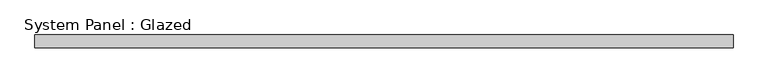
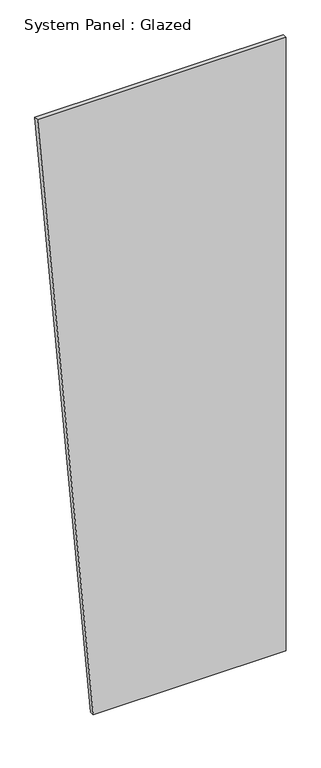
"""IFC4 building model written with IfcOpenShell, lengths in millimetres: plate geometry, System Panel : Glazed."""

import ifcopenshell
import ifcopenshell.guid

model = None  # the IFC model being written
_history = None  # IfcOwnerHistory: only IFC2X3 demands one
_inside = {}  # id of a spatial element -> (the spatial element, [elements in it])
_under = {}  # id of a project, library or spatial element -> (it, [spatial elements below it])
_declared = {}  # id of a project -> (the project, [libraries it declares])
_typed = {}  # id of a type object -> (the type object, [elements of that type])
_made_of = {}  # id of a material, layer set ... -> (it, [elements and type objects made of it])


def new_model(schema):
    """Start an empty IFC model of exactly this schema.

    Asked for "IFC4X3", IfcOpenShell would pick the latest addendum, in which some entities
    have other attributes; the version numbers below select the first issue.
    IFC2X3 requires an IfcOwnerHistory on every rooted entity: one is made here for all.
    """
    global model, _history
    if schema == "IFC4X3":
        model = ifcopenshell.file(schema_version=(4, 3, 0, 0))
    else:
        model = ifcopenshell.file(schema=schema)
    _inside.clear()
    _under.clear()
    _declared.clear()
    _typed.clear()
    _made_of.clear()
    _history = None
    if model.schema == "IFC2X3":
        org = make("IfcOrganization", Name="unknown")
        user = make(
            "IfcPersonAndOrganization",
            ThePerson=make("IfcPerson", FamilyName="unknown"),
            TheOrganization=org,
        )
        app = make(
            "IfcApplication",
            ApplicationDeveloper=org,
            Version="unknown",
            ApplicationFullName="unknown",
            ApplicationIdentifier="unknown",
        )
        _history = make(
            "IfcOwnerHistory",
            OwningUser=user,
            OwningApplication=app,
            ChangeAction="ADDED",
            CreationDate=0,
        )
    return model


def make(cls, **values):
    """One entity of the class cls with the attributes given. An attribute that is None is left unset."""
    return model.create_entity(
        cls, **{name: value for name, value in values.items() if value is not None}
    )


def rooted(cls, **values):
    """An entity with a GlobalId (a new one), such as an element, a storey or a relation."""
    return make(cls, GlobalId=ifcopenshell.guid.new(), OwnerHistory=_history, **values)


def si_unit(unit_type, name, prefix=None):
    """IfcSIUnit, for example si_unit("LENGTHUNIT", "METRE", prefix="MILLI")."""
    return make("IfcSIUnit", UnitType=unit_type, Prefix=prefix, Name=name)


def assignment(units):
    """IfcUnitAssignment: the units of a project."""
    return None if units is None else make("IfcUnitAssignment", Units=units)


def point(xyz):
    """IfcCartesianPoint."""
    return None if xyz is None else make("IfcCartesianPoint", Coordinates=xyz)


def direction(xyz):
    """IfcDirection."""
    return None if xyz is None else make("IfcDirection", DirectionRatios=xyz)


def frame(location, z_axis=None, x_axis=None):
    """IfcAxis2Placement3D, a coordinate frame: its origin and axes. An axis left out is left unset."""
    return make(
        "IfcAxis2Placement3D",
        Location=point(location),
        Axis=direction(z_axis),
        RefDirection=direction(x_axis),
    )


def origin():
    """The frame at (0, 0, 0) with its axes left unset."""
    return frame((0.0, 0.0, 0.0))


def place(relative_to, where):
    """IfcLocalPlacement: puts the frame where relative to a parent placement (None: the world)."""
    return make(
        "IfcLocalPlacement", PlacementRelTo=relative_to, RelativePlacement=where
    )


def context(
    kind, dimensions, precision=None, world=None, true_north=None, identifier=None
):
    """IfcGeometricRepresentationContext, for example the 3D "Model" context."""
    return make(
        "IfcGeometricRepresentationContext",
        ContextIdentifier=identifier,
        ContextType=kind,
        CoordinateSpaceDimension=dimensions,
        Precision=precision,
        WorldCoordinateSystem=world,
        TrueNorth=true_north,
    )


def project(units=None, contexts=None):
    """IfcProject with its units and contexts."""
    return rooted(
        "IfcProject",
        Name="project",
        RepresentationContexts=contexts,
        UnitsInContext=assignment(units),
    )


def spatial(cls, under=None, at=None, **own):
    """A site, building, storey or space (cls), placed at a placement, below another one or the project."""
    s = rooted(cls, ObjectPlacement=at, **own)
    if under is not None:
        _under.setdefault(under.id(), (under, []))[1].append(s)
    return s


def polyline(points):
    """IfcPolyline through the points."""
    return make("IfcPolyline", Points=[point(p) for p in points])


def outline(outer, holes=None, kind="AREA"):
    """IfcArbitraryClosedProfileDef: a profile drawn as a closed curve; with holes, ...WithVoids."""
    if holes is None:
        return make("IfcArbitraryClosedProfileDef", ProfileType=kind, OuterCurve=outer)
    return make(
        "IfcArbitraryProfileDefWithVoids",
        ProfileType=kind,
        OuterCurve=outer,
        InnerCurves=holes,
    )


def extrude(swept, where, along, depth):
    """IfcExtrudedAreaSolid: the profile swept, set in the frame where, extruded along a direction by depth."""
    return make(
        "IfcExtrudedAreaSolid",
        SweptArea=swept,
        Position=where,
        ExtrudedDirection=direction(along),
        Depth=depth,
    )


def shape(context_of_items, identifier, shape_type, items):
    """IfcShapeRepresentation: the items that make up one representation, for example the "Body"."""
    return make(
        "IfcShapeRepresentation",
        ContextOfItems=context_of_items,
        RepresentationIdentifier=identifier,
        RepresentationType=shape_type,
        Items=items,
    )


def source(mapping_origin, context_of_items, identifier, shape_type, items):
    """IfcRepresentationMap: a shape defined once, which mapped items show again and again."""
    return make(
        "IfcRepresentationMap",
        MappingOrigin=mapping_origin,
        MappedRepresentation=shape(context_of_items, identifier, shape_type, items),
    )


def transform(
    local_origin,
    x_axis=None,
    y_axis=None,
    z_axis=None,
    scale=None,
    scale2=None,
    scale3=None,
    uniform=True,
):
    """IfcCartesianTransformationOperator3D, or its non-uniform kind. x_axis, y_axis, z_axis: its Axis1, 2, 3."""
    if uniform:
        return make(
            "IfcCartesianTransformationOperator3D",
            Axis1=direction(x_axis),
            Axis2=direction(y_axis),
            LocalOrigin=point(local_origin),
            Scale=scale,
            Axis3=direction(z_axis),
        )
    return make(
        "IfcCartesianTransformationOperator3DnonUniform",
        Axis1=direction(x_axis),
        Axis2=direction(y_axis),
        LocalOrigin=point(local_origin),
        Scale=scale,
        Axis3=direction(z_axis),
        Scale2=scale2,
        Scale3=scale3,
    )


def mapped(mapping_source, mapping_target):
    """IfcMappedItem: shows the shape of a source again, moved by a transform."""
    return make(
        "IfcMappedItem", MappingSource=mapping_source, MappingTarget=mapping_target
    )


def made_of(thing, what):
    """Note that an element or type object is made of a material, layer set ...; save() writes the relation."""
    if what is not None:
        _made_of.setdefault(what.id(), (what, []))[1].append(thing)
    return thing


def element(
    cls,
    number,
    at=None,
    inside=None,
    cuts=None,
    type_object=None,
    material=None,
    context=None,
    identifier="Body",
    shape_type=None,
    held_by="IfcProductDefinitionShape",
    body=None,
    shapes=None,
    **own,
):
    """One element of the class cls, such as IfcWall. Its Tag is "e" and its number.

    at: its placement. inside: the storey or other place that contains it. cuts: it is an
    opening in that element (IfcRelVoidsElement). A single representation is given by context,
    identifier, shape_type and body (its items); several are given by shapes. held_by: the class
    of the entity that holds the representations. save() writes the other relations.
    """
    e = rooted(cls, Tag="e%d" % number, ObjectPlacement=at, **own)
    if body is not None:
        shapes = [shape(context, identifier, shape_type, body)]
    if shapes is not None:
        e.Representation = make(held_by, Representations=shapes)
    if inside is not None:
        _inside.setdefault(inside.id(), (inside, []))[1].append(e)
    if cuts is not None:
        rooted(
            "IfcRelVoidsElement", RelatingBuildingElement=cuts, RelatedOpeningElement=e
        )
    if type_object is not None:
        _typed.setdefault(type_object.id(), (type_object, []))[1].append(e)
    return made_of(e, material)


def aggregate(whole, parts):
    """IfcRelAggregates: a whole, such as a stair, and the parts it consists of."""
    return rooted("IfcRelAggregates", RelatingObject=whole, RelatedObjects=parts)


def save(model, path):
    """Write the relations noted so far, then the file.

    IfcRelAggregates (storeys below a building ...), IfcRelContainedInSpatialStructure (elements
    in a storey), IfcRelDefinesByType, IfcRelAssociatesMaterial and IfcRelDeclares: one each for
    every whole, place, type object, material and project.
    """
    for whole, parts in _under.values():
        aggregate(whole, parts)
    for where, things in _inside.values():
        rooted(
            "IfcRelContainedInSpatialStructure",
            RelatedElements=things,
            RelatingStructure=where,
        )
    for kind, things in _typed.values():
        rooted("IfcRelDefinesByType", RelatedObjects=things, RelatingType=kind)
    for what, things in _made_of.values():
        rooted("IfcRelAssociatesMaterial", RelatedObjects=things, RelatingMaterial=what)
    for by, libraries in _declared.values():
        rooted("IfcRelDeclares", RelatingContext=by, RelatedDefinitions=libraries)
    model.write(path)


def system_panel_glazed_cde5e94a(model_context):
    return source(origin(), model_context, "Body", "SweptSolid", [
        extrude(outline(polyline([(0.0, -386.1685195), (0.0, 701.3055584), (3657.6, 701.3055584), (3657.6, -701.3055584), (0.0, -386.1685195)])), frame((0.0, -44.45, 0.0), z_axis=(0.0, 1.0, 0.0), x_axis=(0.0, 0.0, 1.0)), (0.0, 0.0, 1.0), 25.4),
    ])


if __name__ == "__main__":
    model = new_model("IFC4")
    model_context = context("Model", 3, world=origin())
    ifc_project = project(units=[si_unit("LENGTHUNIT", "METRE", prefix="MILLI")], contexts=[model_context])
    site = spatial("IfcSite", under=ifc_project)
    building = spatial("IfcBuilding", under=site)
    placement = place(None, origin())
    system_panel_glazed_shape = system_panel_glazed_cde5e94a(model_context)
    element("IfcPlate", 1, ObjectType="System Panel : Glazed", at=placement, inside=building, context=model_context, shape_type="MappedRepresentation", body=[
        mapped(system_panel_glazed_shape, transform((0.0, 0.0, 0.0), x_axis=(1.0, 0.0, 0.0), y_axis=(0.0, 1.0, 0.0), z_axis=(0.0, 0.0, 1.0))),
    ])
    save(model, "model.ifc")

# Revit data of these elements
# Type "System Panel : Glazed"
#   Construction Type Id = "GSP4R"
#   Analytic Construction = "1/8 in Pilkington single glazing"
#   Visual Light Transmittance = 0.9
#   Solar Heat Gain Coefficient = 0.86
#   Heat Transfer Coefficient (U) = 1.18115 BTU/(h·ft²·°F)
#   Define Thermal Properties by = 1
# Element 1 (IfcPlate, "System Panel : Glazed")
#   Materials on its faces: "Glass"
# Materials
#   "Glass": class "Glass", colour RGB 0 128 192, transparency 0.75, Description = "Soda Lime Glass", Cost = 0
